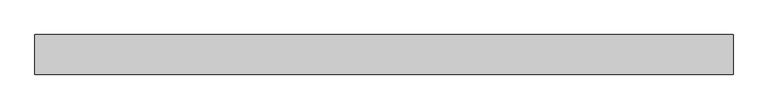
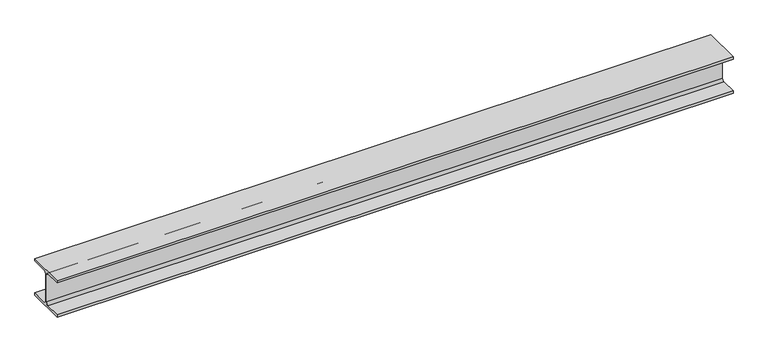
"""IFC4 building model written with IfcOpenShell, lengths in millimetres: beam geometry, 0912_Steel Framing_H-KSD3502 : H_SB_ASB_H-200x200x8x12."""

from ifc_helpers import new_model, si_unit, point, frame, frame_2d, origin, place, context, project, spatial, polyline, circle_curve, trimmed, segment, composite_curve, outline, extrude, source, transform, mapped, element, save


def beam_38e61aa3(model_context):
    return source(origin(), model_context, "Body", "SweptSolid", [
        extrude(outline(composite_curve([segment(polyline([(100.0, -88.0), (100.0, -100.0), (-100.0, -100.0), (-100.0, -88.0), (-17.0, -88.0)]), True, "CONTINUOUS"), segment(trimmed(circle_curve(frame_2d((-17.0, -75.0)), 13.0), [point((-17.0, -88.0))], [point((-4.0, -75.0))], True, "CARTESIAN"), True, "CONTINUOUS"), segment(polyline([(-4.0, -75.0), (-4.0, 75.0)]), True, "CONTINUOUS"), segment(trimmed(circle_curve(frame_2d((-17.0, 75.0)), 13.0), [point((-4.0, 75.0))], [point((-17.0, 88.0))], True, "CARTESIAN"), True, "CONTINUOUS"), segment(polyline([(-17.0, 88.0), (-100.0, 88.0), (-100.0, 100.0), (100.0, 100.0), (100.0, 88.0), (17.0, 88.0)]), True, "CONTINUOUS"), segment(trimmed(circle_curve(frame_2d((17.0, 75.0)), 13.0), [point((17.0, 88.0))], [point((4.0, 75.0))], True, "CARTESIAN"), True, "CONTINUOUS"), segment(polyline([(4.0, 75.0), (4.0, -75.0)]), True, "CONTINUOUS"), segment(trimmed(circle_curve(frame_2d((17.0, -75.0)), 13.0), [point((4.0, -75.0))], [point((17.0, -88.0))], True, "CARTESIAN"), True, "CONTINUOUS"), segment(polyline([(17.0, -88.0), (100.0, -88.0)]), True, "CONTINUOUS")], self_intersect=False)), frame((-1814.5992235, 0.0, 0.0), z_axis=(1.0, 0.0, 0.0), x_axis=(0.0, 1.0, 0.0)), (0.0, 0.0, 1.0), 3525.9751894),
    ])


if __name__ == "__main__":
    model = new_model("IFC4")
    model_context = context("Model", 3, world=origin())
    ifc_project = project(units=[si_unit("LENGTHUNIT", "METRE", prefix="MILLI")], contexts=[model_context])
    site = spatial("IfcSite", under=ifc_project)
    building = spatial("IfcBuilding", under=site)
    placement = place(None, origin())
    beam_shape = beam_38e61aa3(model_context)
    element("IfcBeam", 1, ObjectType="0912_Steel Framing_H-KSD3502 : H_SB_ASB_H-200x200x8x12", at=placement, inside=building, context=model_context, shape_type="MappedRepresentation", body=[
        mapped(beam_shape, transform((0.0, 0.0, 0.0), x_axis=(1.0, 0.0, 0.0), y_axis=(0.0, 1.0, 0.0), z_axis=(0.0, 0.0, 1.0))),
    ])
    save(model, "model.ifc")

# Revit data of these elements
# Type "0912_Steel Framing_H-KSD3502 : H_SB_ASB_H-200x200x8x12"
#   H_WM Code_1 = "S01AA002-00001 | Main Steel Structure Fabrication Work | Shelter/Building | Medium Steel - Standard (90KG/M>Weight≥30KG/M) | Material: (   )"
#   H_WM Code_2 = "S03AA028-00001 | Main Steel Structure Erection Work | Shelter/Building | Medium Steel (90KG/M>Weight≥30KG/M) | Material: (   )"
#   H_WM Code_3 = "S01AA010-00001 | Main Steel Structure Fabrication Work | Shelter/Building | Steel Painting/Coating | for Non-Fireproofed Steel Surface, Surface Preparation, Primer, Second & Final Coat | Material: (   )"
#   H_Q'ty Cal Type Tag = "SB-Q2"
#   Width = 20.0 cm
#   Web Thickness = 0.8 cm
#   Web Fillet = 1.3 cm
#   Warping Constant = 141000.0 cm⁶
#   W = 0
#   Torsional Moment of Inertia = 26.2485 cm⁴
#   Section Area = 63.53 cm²
#   Plastic Modulus weak axis = 244.0 cm³
#   Plastic Modulus strong axis = 525.0 cm³
#   Perimeter = 1.16 m²/m
#   Nominal Weight = 49.90 kgf/m
#   Moment of Inertia weak axis = 1600.00 cm⁴
#   Moment of Inertia strong axis = 4720.00 cm⁴
#   Height = 20.0 cm
#   Flange Thickness = 1.2 cm
#   Elastic Modulus weak axis = 160.0 cm³
#   Elastic Modulus strong axis = 472.0 cm³
#   Centroid Vertical = 10.0 cm
#   Centroid Horizontal = 10.0 cm
#   Ix = 47200000
#   Length [instance default] = 1.5240 m
#   Zx = 525000
#   b = 0.2000 m
#   h = 0.2000 m
#   r = 0.0130 m
#   s = 0.0080 m
#   t = 0.0120 m
#   A = 0.006353 m²
#   Structural Material [instance default] = Steel, 45-345
#   Assembly Code = ""
# Element 1 (IfcBeam, "0912_Steel Framing_H-KSD3502 : H_SB_ASB_H-200x200x8x12")
#   Structural Material = none
# Materials
#   "Steel, 45-345": class "Metal", colour RGB 189 187 185, transparency 0, Description = "Steel 345 MPa", Cost = 0
